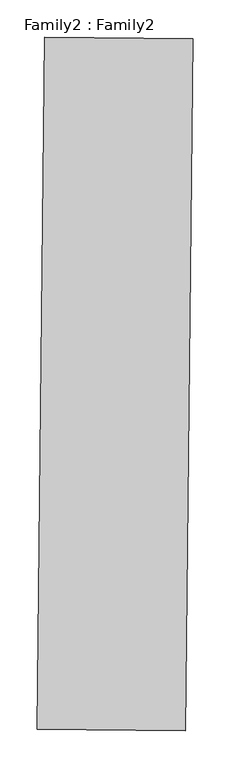
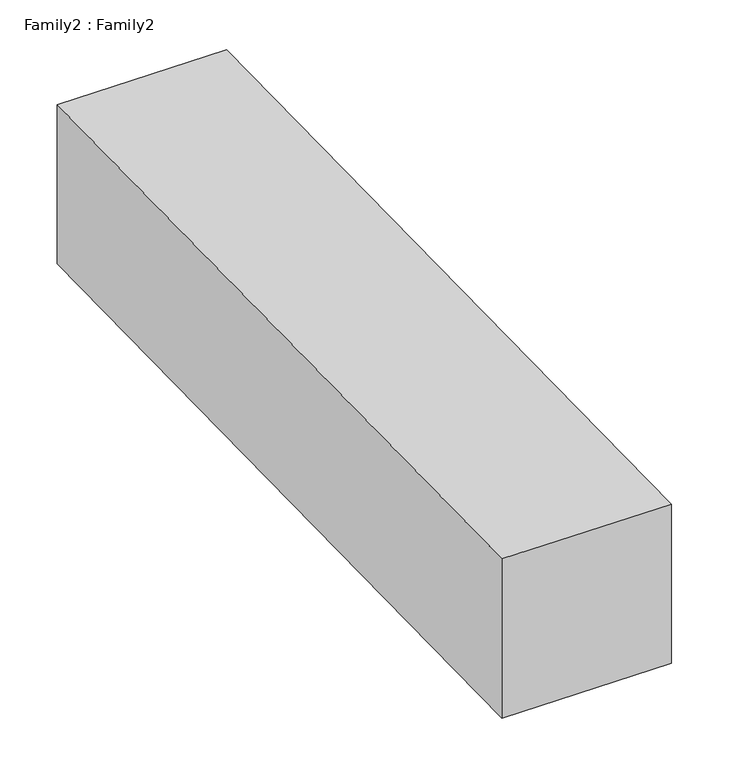
"""IFC4 building model written with IfcOpenShell, lengths in millimetres: proxy geometry, Family2 : Family2."""

from ifc_helpers import new_model, si_unit, origin, place, context, project, spatial, faceted_brep, source, transform, mapped, element, save


def family2_family2_5f336d8f(model_context):
    return source(origin(), model_context, "Body", "Brep", [
        faceted_brep([(-3948.6111591, -6539.9163554, 1.0945136), (-3948.6111591, -6539.9163554, 201.0945136), (-3938.2316354, -5607.6837672, 202.060409), (-3938.2316354, -5607.6837672, 2.060409), (-3748.6199692, -6541.7935681, 201.0945136), (-3738.2404454, -5609.5609798, 202.060409), (-3748.6199692, -6541.7935681, 1.0945136), (-3738.2404454, -5609.5609798, 2.060409)], [[[0, 1, 2, 3]], [[1, 4, 5, 2]], [[4, 6, 7, 5]], [[6, 0, 3, 7]], [[3, 2, 5, 7]], [[0, 6, 4, 1]]]),
    ])


if __name__ == "__main__":
    model = new_model("IFC4")
    model_context = context("Model", 3, world=origin())
    ifc_project = project(units=[si_unit("LENGTHUNIT", "METRE", prefix="MILLI")], contexts=[model_context])
    site = spatial("IfcSite", under=ifc_project)
    building = spatial("IfcBuilding", under=site)
    placement = place(None, origin())
    family2_family2_shape = family2_family2_5f336d8f(model_context)
    element("IfcBuildingElementProxy", 1, Name="Family2 : Family2", ObjectType="Family2 : Family2", at=placement, inside=building, context=model_context, shape_type="MappedRepresentation", body=[
        mapped(family2_family2_shape, transform((0.0, 0.0, 0.0), x_axis=(1.0, 0.0, 0.0), y_axis=(0.0, 1.0, 0.0), z_axis=(0.0, 0.0, 1.0))),
    ])
    save(model, "model.ifc")

# Revit data of these elements
# Type "Family2 : Family2"
#   Default Elevation = 0
